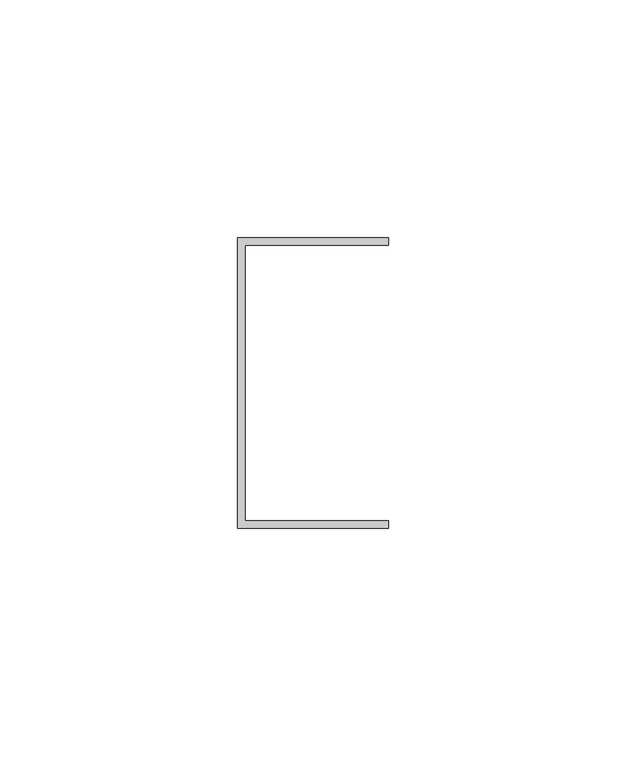
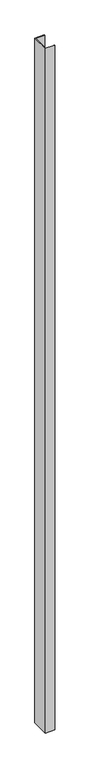
"""IFC4 building model written with IfcOpenShell, lengths in millimetres: proxy geometry, Generic Models 7:Generic Models 1:3:Generic Models 1:3 : Generic Models 7:Generic Models 1:305549:3:Generic Models 1:3:Generic Models 1:3 : Generic Models 7:Generic Models 1:305549:3 : Generic Models 7:Generic Models 1:3:Generic Models 1:3 : Generic Models 7:Generic Models 1:305549:301244:4 : Generic Models 7:Generic Models 1:3:Generic Models 1:3 : Generic Models 7:Generic Models 1:305549:3:Generic Models 1:3:Generic Models 1:3 : Generic Models 7:Generic Models 1:305549:3 : Generic Models 7:Generic Models 1:3:Generic Models 1:3 : Generic Models 7:Generic Models 1:305549:301244:308848."""

import ifcopenshell
import ifcopenshell.guid

model = None  # the IFC model being written
_history = None  # IfcOwnerHistory: only IFC2X3 demands one
_inside = {}  # id of a spatial element -> (the spatial element, [elements in it])
_under = {}  # id of a project, library or spatial element -> (it, [spatial elements below it])
_declared = {}  # id of a project -> (the project, [libraries it declares])
_typed = {}  # id of a type object -> (the type object, [elements of that type])
_made_of = {}  # id of a material, layer set ... -> (it, [elements and type objects made of it])


def new_model(schema):
    """Start an empty IFC model of exactly this schema.

    Asked for "IFC4X3", IfcOpenShell would pick the latest addendum, in which some entities
    have other attributes; the version numbers below select the first issue.
    IFC2X3 requires an IfcOwnerHistory on every rooted entity: one is made here for all.
    """
    global model, _history
    if schema == "IFC4X3":
        model = ifcopenshell.file(schema_version=(4, 3, 0, 0))
    else:
        model = ifcopenshell.file(schema=schema)
    _inside.clear()
    _under.clear()
    _declared.clear()
    _typed.clear()
    _made_of.clear()
    _history = None
    if model.schema == "IFC2X3":
        org = make("IfcOrganization", Name="unknown")
        user = make(
            "IfcPersonAndOrganization",
            ThePerson=make("IfcPerson", FamilyName="unknown"),
            TheOrganization=org,
        )
        app = make(
            "IfcApplication",
            ApplicationDeveloper=org,
            Version="unknown",
            ApplicationFullName="unknown",
            ApplicationIdentifier="unknown",
        )
        _history = make(
            "IfcOwnerHistory",
            OwningUser=user,
            OwningApplication=app,
            ChangeAction="ADDED",
            CreationDate=0,
        )
    return model


def make(cls, **values):
    """One entity of the class cls with the attributes given. An attribute that is None is left unset."""
    return model.create_entity(
        cls, **{name: value for name, value in values.items() if value is not None}
    )


def rooted(cls, **values):
    """An entity with a GlobalId (a new one), such as an element, a storey or a relation."""
    return make(cls, GlobalId=ifcopenshell.guid.new(), OwnerHistory=_history, **values)


def si_unit(unit_type, name, prefix=None):
    """IfcSIUnit, for example si_unit("LENGTHUNIT", "METRE", prefix="MILLI")."""
    return make("IfcSIUnit", UnitType=unit_type, Prefix=prefix, Name=name)


def assignment(units):
    """IfcUnitAssignment: the units of a project."""
    return None if units is None else make("IfcUnitAssignment", Units=units)


def point(xyz):
    """IfcCartesianPoint."""
    return None if xyz is None else make("IfcCartesianPoint", Coordinates=xyz)


def direction(xyz):
    """IfcDirection."""
    return None if xyz is None else make("IfcDirection", DirectionRatios=xyz)


def frame(location, z_axis=None, x_axis=None):
    """IfcAxis2Placement3D, a coordinate frame: its origin and axes. An axis left out is left unset."""
    return make(
        "IfcAxis2Placement3D",
        Location=point(location),
        Axis=direction(z_axis),
        RefDirection=direction(x_axis),
    )


def origin():
    """The frame at (0, 0, 0) with its axes left unset."""
    return frame((0.0, 0.0, 0.0))


def place(relative_to, where):
    """IfcLocalPlacement: puts the frame where relative to a parent placement (None: the world)."""
    return make(
        "IfcLocalPlacement", PlacementRelTo=relative_to, RelativePlacement=where
    )


def context(
    kind, dimensions, precision=None, world=None, true_north=None, identifier=None
):
    """IfcGeometricRepresentationContext, for example the 3D "Model" context."""
    return make(
        "IfcGeometricRepresentationContext",
        ContextIdentifier=identifier,
        ContextType=kind,
        CoordinateSpaceDimension=dimensions,
        Precision=precision,
        WorldCoordinateSystem=world,
        TrueNorth=true_north,
    )


def project(units=None, contexts=None):
    """IfcProject with its units and contexts."""
    return rooted(
        "IfcProject",
        Name="project",
        RepresentationContexts=contexts,
        UnitsInContext=assignment(units),
    )


def spatial(cls, under=None, at=None, **own):
    """A site, building, storey or space (cls), placed at a placement, below another one or the project."""
    s = rooted(cls, ObjectPlacement=at, **own)
    if under is not None:
        _under.setdefault(under.id(), (under, []))[1].append(s)
    return s


def polyline(points):
    """IfcPolyline through the points."""
    return make("IfcPolyline", Points=[point(p) for p in points])


def outline(outer, holes=None, kind="AREA"):
    """IfcArbitraryClosedProfileDef: a profile drawn as a closed curve; with holes, ...WithVoids."""
    if holes is None:
        return make("IfcArbitraryClosedProfileDef", ProfileType=kind, OuterCurve=outer)
    return make(
        "IfcArbitraryProfileDefWithVoids",
        ProfileType=kind,
        OuterCurve=outer,
        InnerCurves=holes,
    )


def extrude(swept, where, along, depth):
    """IfcExtrudedAreaSolid: the profile swept, set in the frame where, extruded along a direction by depth."""
    return make(
        "IfcExtrudedAreaSolid",
        SweptArea=swept,
        Position=where,
        ExtrudedDirection=direction(along),
        Depth=depth,
    )


def shape(context_of_items, identifier, shape_type, items):
    """IfcShapeRepresentation: the items that make up one representation, for example the "Body"."""
    return make(
        "IfcShapeRepresentation",
        ContextOfItems=context_of_items,
        RepresentationIdentifier=identifier,
        RepresentationType=shape_type,
        Items=items,
    )


def source(mapping_origin, context_of_items, identifier, shape_type, items):
    """IfcRepresentationMap: a shape defined once, which mapped items show again and again."""
    return make(
        "IfcRepresentationMap",
        MappingOrigin=mapping_origin,
        MappedRepresentation=shape(context_of_items, identifier, shape_type, items),
    )


def transform(
    local_origin,
    x_axis=None,
    y_axis=None,
    z_axis=None,
    scale=None,
    scale2=None,
    scale3=None,
    uniform=True,
):
    """IfcCartesianTransformationOperator3D, or its non-uniform kind. x_axis, y_axis, z_axis: its Axis1, 2, 3."""
    if uniform:
        return make(
            "IfcCartesianTransformationOperator3D",
            Axis1=direction(x_axis),
            Axis2=direction(y_axis),
            LocalOrigin=point(local_origin),
            Scale=scale,
            Axis3=direction(z_axis),
        )
    return make(
        "IfcCartesianTransformationOperator3DnonUniform",
        Axis1=direction(x_axis),
        Axis2=direction(y_axis),
        LocalOrigin=point(local_origin),
        Scale=scale,
        Axis3=direction(z_axis),
        Scale2=scale2,
        Scale3=scale3,
    )


def mapped(mapping_source, mapping_target):
    """IfcMappedItem: shows the shape of a source again, moved by a transform."""
    return make(
        "IfcMappedItem", MappingSource=mapping_source, MappingTarget=mapping_target
    )


def made_of(thing, what):
    """Note that an element or type object is made of a material, layer set ...; save() writes the relation."""
    if what is not None:
        _made_of.setdefault(what.id(), (what, []))[1].append(thing)
    return thing


def element(
    cls,
    number,
    at=None,
    inside=None,
    cuts=None,
    type_object=None,
    material=None,
    context=None,
    identifier="Body",
    shape_type=None,
    held_by="IfcProductDefinitionShape",
    body=None,
    shapes=None,
    **own,
):
    """One element of the class cls, such as IfcWall. Its Tag is "e" and its number.

    at: its placement. inside: the storey or other place that contains it. cuts: it is an
    opening in that element (IfcRelVoidsElement). A single representation is given by context,
    identifier, shape_type and body (its items); several are given by shapes. held_by: the class
    of the entity that holds the representations. save() writes the other relations.
    """
    e = rooted(cls, Tag="e%d" % number, ObjectPlacement=at, **own)
    if body is not None:
        shapes = [shape(context, identifier, shape_type, body)]
    if shapes is not None:
        e.Representation = make(held_by, Representations=shapes)
    if inside is not None:
        _inside.setdefault(inside.id(), (inside, []))[1].append(e)
    if cuts is not None:
        rooted(
            "IfcRelVoidsElement", RelatingBuildingElement=cuts, RelatedOpeningElement=e
        )
    if type_object is not None:
        _typed.setdefault(type_object.id(), (type_object, []))[1].append(e)
    return made_of(e, material)


def aggregate(whole, parts):
    """IfcRelAggregates: a whole, such as a stair, and the parts it consists of."""
    return rooted("IfcRelAggregates", RelatingObject=whole, RelatedObjects=parts)


def save(model, path):
    """Write the relations noted so far, then the file.

    IfcRelAggregates (storeys below a building ...), IfcRelContainedInSpatialStructure (elements
    in a storey), IfcRelDefinesByType, IfcRelAssociatesMaterial and IfcRelDeclares: one each for
    every whole, place, type object, material and project.
    """
    for whole, parts in _under.values():
        aggregate(whole, parts)
    for where, things in _inside.values():
        rooted(
            "IfcRelContainedInSpatialStructure",
            RelatedElements=things,
            RelatingStructure=where,
        )
    for kind, things in _typed.values():
        rooted("IfcRelDefinesByType", RelatedObjects=things, RelatingType=kind)
    for what, things in _made_of.values():
        rooted("IfcRelAssociatesMaterial", RelatedObjects=things, RelatingMaterial=what)
    for by, libraries in _declared.values():
        rooted("IfcRelDeclares", RelatingContext=by, RelatedDefinitions=libraries)
    model.write(path)


def generic_models_d8cc08ce(model_context):
    return source(origin(), model_context, "Body", "SweptSolid", [
        extrude(outline(polyline([(594982.6867239, -579015.772634), (595014.4367239, -579015.772634), (595014.4367239, -579017.360134), (594984.2742239, -579017.360134), (594984.2742239, -579075.303884), (595014.4367239, -579075.303884), (595014.4367239, -579076.891384), (594982.6867239, -579076.891384), (594982.6867239, -579015.772634)])), frame((0.0, 0.0, 50.8), z_axis=(0.0, 0.0, 1.0), x_axis=(1.0, 0.0, 0.0)), (0.0, 0.0, 1.0), 2430.9324376),
    ])


if __name__ == "__main__":
    model = new_model("IFC4")
    model_context = context("Model", 3, world=origin())
    ifc_project = project(units=[si_unit("LENGTHUNIT", "METRE", prefix="MILLI")], contexts=[model_context])
    site = spatial("IfcSite", under=ifc_project)
    building = spatial("IfcBuilding", under=site)
    placement = place(None, origin())
    generic_models_shape = generic_models_d8cc08ce(model_context)
    element("IfcBuildingElementProxy", 1, Name="Generic Models 7:Generic Models 1:3:Generic Models 1:3 : Generic Models 7:Generic Models 1:305549:3:Generic Models 1:3:Generic Models 1:3 : Generic Models 7:Generic Models 1:305549:3 : Generic Models 7:Generic Models 1:3:Generic Models 1:3 : Generic Models 7:Generic Models 1:305549:301244:4 : Generic Models 7:Generic Models 1:3:Generic Models 1:3 : Generic Models 7:Generic Models 1:305549:3:Generic Models 1:3:Generic Models 1:3 : Generic Models 7:Generic Models 1:305549:3 : Generic Models 7:Generic Models 1:3:Generic Models 1:3 : Generic Models 7:Generic Models 1:305549:301244:308848", ObjectType="Generic Models 7:Generic Models 1:3:Generic Models 1:3 : Generic Models 7:Generic Models 1:305549:3:Generic Models 1:3:Generic Models 1:3 : Generic Models 7:Generic Models 1:305549:3 : Generic Models 7:Generic Models 1:3:Generic Models 1:3 : Generic Models 7:Generic Models 1:305549:301244:4 : Generic Models 7:Generic Models 1:3:Generic Models 1:3 : Generic Models 7:Generic Models 1:305549:3:Generic Models 1:3:Generic Models 1:3 : Generic Models 7:Generic Models 1:305549:3 : Generic Models 7:Generic Models 1:3:Generic Models 1:3 : Generic Models 7:Generic Models 1:305549:301244:308848", at=placement, inside=building, context=model_context, shape_type="MappedRepresentation", body=[
        mapped(generic_models_shape, transform((0.0, 0.0, 0.0), x_axis=(1.0, 0.0, 0.0), y_axis=(0.0, 1.0, 0.0), z_axis=(0.0, 0.0, 1.0))),
    ])
    save(model, "model.ifc")

# Revit data of these elements
# Type "Generic Models 7:Generic Models 1:3:Generic Models 1:3 : Generic Models 7:Generic Models 1:305549:3:Generic Models 1:3:Generic Models 1:3 : Generic Models 7:Generic Models 1:305549:3 : Generic Models 7:Generic Models 1:3:Generic Models 1:3 : Generic Models 7:Generic Models 1:305549:301244:4 : Generic Models 7:Generic Models 1:3:Generic Models 1:3 : Generic Models 7:Generic Models 1:305549:3:Generic Models 1:3:Generic Models 1:3 : Generic Models 7:Generic Models 1:305549:3 : Generic Models 7:Generic Models 1:3:Generic Models 1:3 : Generic Models 7:Generic Models 1:305549:301244:308848"
#   NameOverride = "Generic Models 7:Generic Models 1:3:Generic Models 1:3 : Generic Models 7:Generic Models 1:305549:3:Generic Models 1:3:Generic Models 1:3 : Generic Models 7:Generic Models 1:305549:3 : Generic Models 7:Generic Models 1:3:Generic Models 1:3 : Generic Models 7:Generic Models 1:305549:301244:308848"
#   ObjectTypeOverride = "Generic Models 1:3:Generic Models 1:3 : Generic Models 7:Generic Models 1:305549:3 : Generic Models 7:Generic Models 1:3:Generic Models 1:3 : Generic Models 7:Generic Models 1:305549:301244"
#   Reference = "Generic Models 1"
#   Tag = "308848"
# Element 1 (IfcBuildingElementProxy, "Generic Models 7:Generic Models 1:3:Generic Models 1:3 : Generic Models 7:Generic Models 1:305549:3:Generic Models 1:3:Generic Models 1:3 : Generic Models 7:Generic Models 1:305549:3 : Generic Models 7:Generic Models 1:3:Generic Models 1:3 : Generic Models 7:Generic Models 1:305549:301244:4 : Generic Models 7:Generic Models 1:3:Generic Models 1:3 : Generic Models 7:Generic Models 1:305549:3:Generic Models 1:3:Generic Models 1:3 : Generic Models 7:Generic Models 1:305549:3 : Generic Models 7:Generic Models 1:3:Generic Models 1:3 : Generic Models 7:Generic Models 1:305549:301244:308848")
#   Materials on its faces: "GALVANIZED U-CHANNEL (250T125-33)"
# Materials
#   "GALVANIZED U-CHANNEL (250T125-33)": class "Unassigned", colour RGB 202 201 200, transparency 0, Keynote = "M05451300.02", Cost = 0
